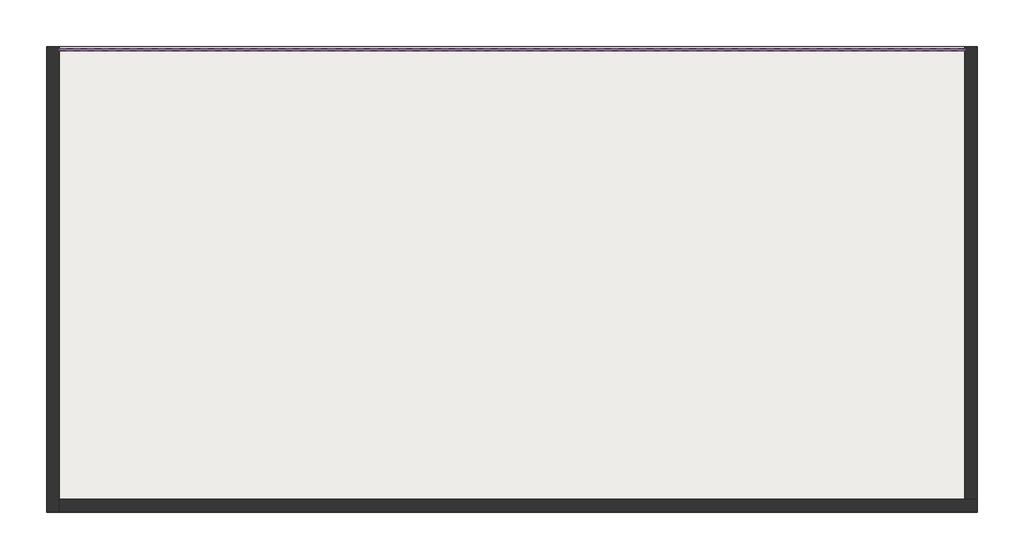
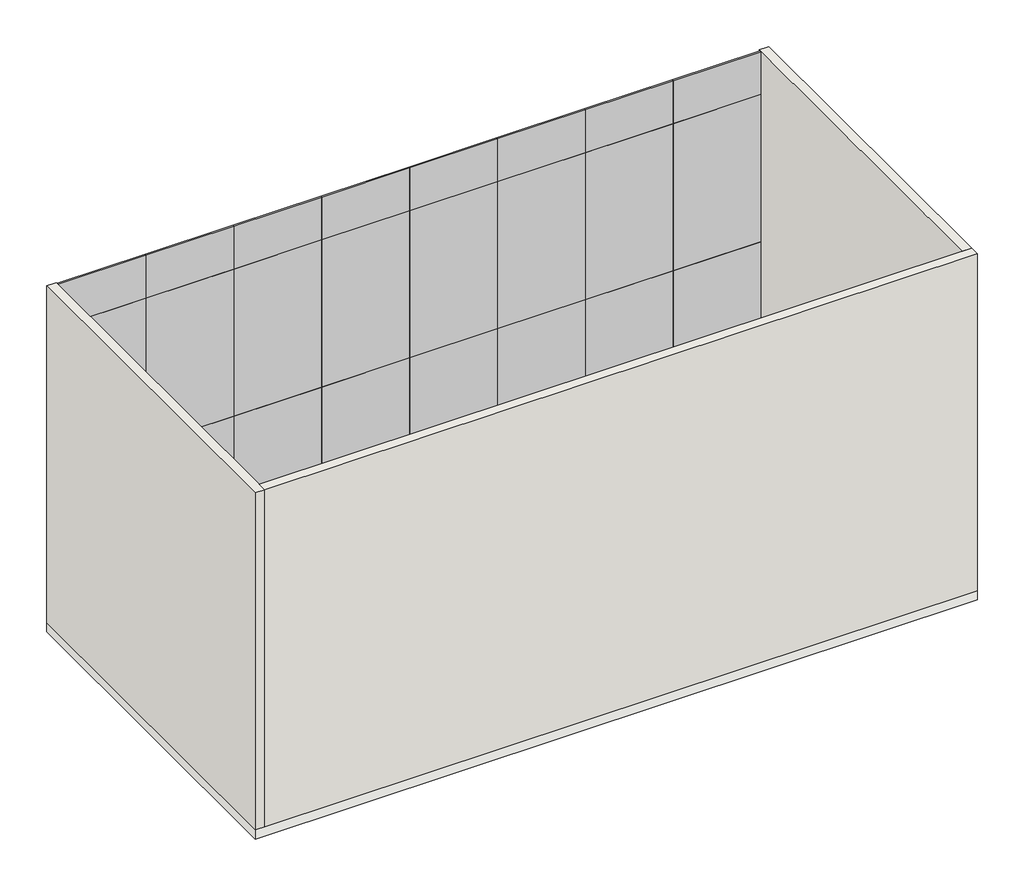
# One storey: 24 plates, 3 walls, 1 slab.
"""IFC4 building model written with IfcOpenShell, lengths in millimetres."""

import ifcopenshell
import ifcopenshell.guid

model = None  # the IFC model being written
_history = None  # IfcOwnerHistory: only IFC2X3 demands one
_inside = {}  # id of a spatial element -> (the spatial element, [elements in it])
_under = {}  # id of a project, library or spatial element -> (it, [spatial elements below it])
_declared = {}  # id of a project -> (the project, [libraries it declares])
_typed = {}  # id of a type object -> (the type object, [elements of that type])
_made_of = {}  # id of a material, layer set ... -> (it, [elements and type objects made of it])


def new_model(schema):
    """Start an empty IFC model of exactly this schema.

    Asked for "IFC4X3", IfcOpenShell would pick the latest addendum, in which some entities
    have other attributes; the version numbers below select the first issue.
    IFC2X3 requires an IfcOwnerHistory on every rooted entity: one is made here for all.
    """
    global model, _history
    if schema == "IFC4X3":
        model = ifcopenshell.file(schema_version=(4, 3, 0, 0))
    else:
        model = ifcopenshell.file(schema=schema)
    _inside.clear()
    _under.clear()
    _declared.clear()
    _typed.clear()
    _made_of.clear()
    _history = None
    if model.schema == "IFC2X3":
        org = make("IfcOrganization", Name="unknown")
        user = make(
            "IfcPersonAndOrganization",
            ThePerson=make("IfcPerson", FamilyName="unknown"),
            TheOrganization=org,
        )
        app = make(
            "IfcApplication",
            ApplicationDeveloper=org,
            Version="unknown",
            ApplicationFullName="unknown",
            ApplicationIdentifier="unknown",
        )
        _history = make(
            "IfcOwnerHistory",
            OwningUser=user,
            OwningApplication=app,
            ChangeAction="ADDED",
            CreationDate=0,
        )
    return model


def make(cls, **values):
    """One entity of the class cls with the attributes given. An attribute that is None is left unset."""
    return model.create_entity(
        cls, **{name: value for name, value in values.items() if value is not None}
    )


def rooted(cls, **values):
    """An entity with a GlobalId (a new one), such as an element, a storey or a relation."""
    return make(cls, GlobalId=ifcopenshell.guid.new(), OwnerHistory=_history, **values)


def si_unit(unit_type, name, prefix=None):
    """IfcSIUnit, for example si_unit("LENGTHUNIT", "METRE", prefix="MILLI")."""
    return make("IfcSIUnit", UnitType=unit_type, Prefix=prefix, Name=name)


def assignment(units):
    """IfcUnitAssignment: the units of a project."""
    return None if units is None else make("IfcUnitAssignment", Units=units)


def point(xyz):
    """IfcCartesianPoint."""
    return None if xyz is None else make("IfcCartesianPoint", Coordinates=xyz)


def direction(xyz):
    """IfcDirection."""
    return None if xyz is None else make("IfcDirection", DirectionRatios=xyz)


def frame(location, z_axis=None, x_axis=None):
    """IfcAxis2Placement3D, a coordinate frame: its origin and axes. An axis left out is left unset."""
    return make(
        "IfcAxis2Placement3D",
        Location=point(location),
        Axis=direction(z_axis),
        RefDirection=direction(x_axis),
    )


def origin():
    """The frame at (0, 0, 0) with its axes left unset."""
    return frame((0.0, 0.0, 0.0))


def origin_with_axes():
    """The frame at (0, 0, 0) with the z axis (0, 0, 1) and the x axis (1, 0, 0) written out."""
    return frame((0.0, 0.0, 0.0), z_axis=(0.0, 0.0, 1.0), x_axis=(1.0, 0.0, 0.0))


def place(relative_to, where):
    """IfcLocalPlacement: puts the frame where relative to a parent placement (None: the world)."""
    return make(
        "IfcLocalPlacement", PlacementRelTo=relative_to, RelativePlacement=where
    )


def context(
    kind, dimensions, precision=None, world=None, true_north=None, identifier=None
):
    """IfcGeometricRepresentationContext, for example the 3D "Model" context."""
    return make(
        "IfcGeometricRepresentationContext",
        ContextIdentifier=identifier,
        ContextType=kind,
        CoordinateSpaceDimension=dimensions,
        Precision=precision,
        WorldCoordinateSystem=world,
        TrueNorth=true_north,
    )


def project(units=None, contexts=None):
    """IfcProject with its units and contexts."""
    return rooted(
        "IfcProject",
        Name="project",
        RepresentationContexts=contexts,
        UnitsInContext=assignment(units),
    )


def spatial(cls, under=None, at=None, **own):
    """A site, building, storey or space (cls), placed at a placement, below another one or the project."""
    s = rooted(cls, ObjectPlacement=at, **own)
    if under is not None:
        _under.setdefault(under.id(), (under, []))[1].append(s)
    return s


def polyline(points):
    """IfcPolyline through the points."""
    return make("IfcPolyline", Points=[point(p) for p in points])


def outline(outer, holes=None, kind="AREA"):
    """IfcArbitraryClosedProfileDef: a profile drawn as a closed curve; with holes, ...WithVoids."""
    if holes is None:
        return make("IfcArbitraryClosedProfileDef", ProfileType=kind, OuterCurve=outer)
    return make(
        "IfcArbitraryProfileDefWithVoids",
        ProfileType=kind,
        OuterCurve=outer,
        InnerCurves=holes,
    )


def extrude(swept, where, along, depth):
    """IfcExtrudedAreaSolid: the profile swept, set in the frame where, extruded along a direction by depth."""
    return make(
        "IfcExtrudedAreaSolid",
        SweptArea=swept,
        Position=where,
        ExtrudedDirection=direction(along),
        Depth=depth,
    )


def faces_of(points, faces, orient=None, outer=None):
    """IfcFace entities. A face is a list of loops; a loop is a list of indices into points, from 0.

    orient and outer hold one flag for each loop. By default every Orientation is true, the
    first loop of a face is its IfcFaceOuterBound and the others are IfcFaceBound.
    """
    made = []
    for i, loops in enumerate(faces):
        bounds = []
        for j, loop in enumerate(loops):
            is_outer = j == 0 if outer is None else outer[i][j]
            bounds.append(
                make(
                    "IfcFaceOuterBound" if is_outer else "IfcFaceBound",
                    Bound=make("IfcPolyLoop", Polygon=[points[k] for k in loop]),
                    Orientation=True if orient is None else orient[i][j],
                )
            )
        made.append(make("IfcFace", Bounds=bounds))
    return made


def faceted_brep(points, faces, orient=None, outer=None, voids=None):
    """IfcFacetedBrep: a solid bounded by flat faces; with voids (closed shells), ...WithVoids."""
    shared = [point(p) for p in points]
    hull = make("IfcClosedShell", CfsFaces=faces_of(shared, faces, orient, outer))
    if voids is None:
        return make("IfcFacetedBrep", Outer=hull)
    return make(
        "IfcFacetedBrepWithVoids",
        Outer=hull,
        Voids=[
            make(cls, CfsFaces=faces_of(shared, fs, o, b)) for cls, fs, o, b in voids
        ],
    )


def shape(context_of_items, identifier, shape_type, items):
    """IfcShapeRepresentation: the items that make up one representation, for example the "Body"."""
    return make(
        "IfcShapeRepresentation",
        ContextOfItems=context_of_items,
        RepresentationIdentifier=identifier,
        RepresentationType=shape_type,
        Items=items,
    )


def source(mapping_origin, context_of_items, identifier, shape_type, items):
    """IfcRepresentationMap: a shape defined once, which mapped items show again and again."""
    return make(
        "IfcRepresentationMap",
        MappingOrigin=mapping_origin,
        MappedRepresentation=shape(context_of_items, identifier, shape_type, items),
    )


def transform(
    local_origin,
    x_axis=None,
    y_axis=None,
    z_axis=None,
    scale=None,
    scale2=None,
    scale3=None,
    uniform=True,
):
    """IfcCartesianTransformationOperator3D, or its non-uniform kind. x_axis, y_axis, z_axis: its Axis1, 2, 3."""
    if uniform:
        return make(
            "IfcCartesianTransformationOperator3D",
            Axis1=direction(x_axis),
            Axis2=direction(y_axis),
            LocalOrigin=point(local_origin),
            Scale=scale,
            Axis3=direction(z_axis),
        )
    return make(
        "IfcCartesianTransformationOperator3DnonUniform",
        Axis1=direction(x_axis),
        Axis2=direction(y_axis),
        LocalOrigin=point(local_origin),
        Scale=scale,
        Axis3=direction(z_axis),
        Scale2=scale2,
        Scale3=scale3,
    )


def mapped(mapping_source, mapping_target):
    """IfcMappedItem: shows the shape of a source again, moved by a transform."""
    return make(
        "IfcMappedItem", MappingSource=mapping_source, MappingTarget=mapping_target
    )


def made_of(thing, what):
    """Note that an element or type object is made of a material, layer set ...; save() writes the relation."""
    if what is not None:
        _made_of.setdefault(what.id(), (what, []))[1].append(thing)
    return thing


def element(
    cls,
    number,
    at=None,
    inside=None,
    cuts=None,
    type_object=None,
    material=None,
    context=None,
    identifier="Body",
    shape_type=None,
    held_by="IfcProductDefinitionShape",
    body=None,
    shapes=None,
    **own,
):
    """One element of the class cls, such as IfcWall. Its Tag is "e" and its number.

    at: its placement. inside: the storey or other place that contains it. cuts: it is an
    opening in that element (IfcRelVoidsElement). A single representation is given by context,
    identifier, shape_type and body (its items); several are given by shapes. held_by: the class
    of the entity that holds the representations. save() writes the other relations.
    """
    e = rooted(cls, Tag="e%d" % number, ObjectPlacement=at, **own)
    if body is not None:
        shapes = [shape(context, identifier, shape_type, body)]
    if shapes is not None:
        e.Representation = make(held_by, Representations=shapes)
    if inside is not None:
        _inside.setdefault(inside.id(), (inside, []))[1].append(e)
    if cuts is not None:
        rooted(
            "IfcRelVoidsElement", RelatingBuildingElement=cuts, RelatedOpeningElement=e
        )
    if type_object is not None:
        _typed.setdefault(type_object.id(), (type_object, []))[1].append(e)
    return made_of(e, material)


def aggregate(whole, parts):
    """IfcRelAggregates: a whole, such as a stair, and the parts it consists of."""
    return rooted("IfcRelAggregates", RelatingObject=whole, RelatedObjects=parts)


def save(model, path):
    """Write the relations noted so far, then the file.

    IfcRelAggregates (storeys below a building ...), IfcRelContainedInSpatialStructure (elements
    in a storey), IfcRelDefinesByType, IfcRelAssociatesMaterial and IfcRelDeclares: one each for
    every whole, place, type object, material and project.
    """
    for whole, parts in _under.values():
        aggregate(whole, parts)
    for where, things in _inside.values():
        rooted(
            "IfcRelContainedInSpatialStructure",
            RelatedElements=things,
            RelatingStructure=where,
        )
    for kind, things in _typed.values():
        rooted("IfcRelDefinesByType", RelatedObjects=things, RelatingType=kind)
    for what, things in _made_of.values():
        rooted("IfcRelAssociatesMaterial", RelatedObjects=things, RelatingMaterial=what)
    for by, libraries in _declared.values():
        rooted("IfcRelDeclares", RelatingContext=by, RelatedDefinitions=libraries)
    model.write(path)


def plate_c1c025ea(model_context):
    return source(origin(), model_context, "Body", "SweptSolid", [
        extrude(outline(polyline([(678.1250001, 24.5), (-678.1250001, 24.5), (-678.1250001, 49.5), (678.1250001, 49.5), (678.1250001, 24.5)])), origin_with_axes(), (0.0, 0.0, 1.0), 2400.0),
    ])


def plate_0eebf7e9(model_context):
    return source(origin(), model_context, "Body", "SweptSolid", [
        extrude(outline(polyline([(678.1250001, 24.5), (-678.1250001, 24.5), (-678.1250001, 49.5), (678.1250001, 49.5), (678.1250001, 24.5)])), origin_with_axes(), (0.0, 0.0, 1.0), 700.0),
    ])


model = new_model("IFC4")

# Units and contexts
model_context = context("Model", 3, world=origin())
ifc_project = project(units=[si_unit("LENGTHUNIT", "METRE", prefix="MILLI")], contexts=[model_context])

# Site, building, storey
site = spatial("IfcSite", under=ifc_project)
building = spatial("IfcBuilding", under=site)
storey = spatial("IfcBuildingStorey", under=building, Name="レベル 1", Elevation=500.0)

# Plates
placement = place(None, origin())
plate_shape = plate_c1c025ea(model_context)
element("IfcPlate", 1, ObjectType="システム パネル : ガラス", at=placement, inside=storey, context=model_context, shape_type="MappedRepresentation", body=[
    mapped(plate_shape, transform((2064.186127, 4477.4867718, 500.0), x_axis=(-1.0, 0.0, 0.0), y_axis=(0.0, -1.0, 0.0), z_axis=(0.0, 0.0, 1.0))),
])
element("IfcPlate", 2, ObjectType="システム パネル : ガラス", at=placement, inside=storey, context=model_context, shape_type="MappedRepresentation", body=[
    mapped(plate_shape, transform((707.9361269, 4477.4867718, 500.0), x_axis=(-1.0, 0.0, 0.0), y_axis=(0.0, -1.0, 0.0), z_axis=(0.0, 0.0, 1.0))),
])
element("IfcPlate", 3, ObjectType="システム パネル : ガラス", at=placement, inside=storey, context=model_context, shape_type="MappedRepresentation", body=[
    mapped(plate_shape, transform((-648.313873, 4477.4867718, 500.0), x_axis=(-1.0, 0.0, 0.0), y_axis=(0.0, -1.0, 0.0), z_axis=(0.0, 0.0, 1.0))),
])
element("IfcPlate", 4, ObjectType="システム パネル : ガラス", at=placement, inside=storey, context=model_context, shape_type="MappedRepresentation", body=[
    mapped(plate_shape, transform((-2004.5638729, 4477.4867718, 500.0), x_axis=(-1.0, 0.0, 0.0), y_axis=(0.0, -1.0, 0.0), z_axis=(0.0, 0.0, 1.0))),
])
element("IfcPlate", 5, ObjectType="システム パネル : ガラス", at=placement, inside=storey, context=model_context, shape_type="MappedRepresentation", body=[
    mapped(plate_shape, transform((-3360.8138728, 4477.4867718, 500.0), x_axis=(-1.0, 0.0, 0.0), y_axis=(0.0, -1.0, 0.0), z_axis=(0.0, 0.0, 1.0))),
])
element("IfcPlate", 6, ObjectType="システム パネル : ガラス", at=placement, inside=storey, context=model_context, shape_type="MappedRepresentation", body=[
    mapped(plate_shape, transform((-4717.0638727, 4477.4867718, 500.0), x_axis=(-1.0, 0.0, 0.0), y_axis=(0.0, -1.0, 0.0), z_axis=(0.0, 0.0, 1.0))),
])
element("IfcPlate", 7, ObjectType="システム パネル : ガラス", at=placement, inside=storey, context=model_context, shape_type="MappedRepresentation", body=[
    mapped(plate_shape, transform((-6073.3138727, 4477.4867718, 500.0), x_axis=(-1.0, 0.0, 0.0), y_axis=(0.0, -1.0, 0.0), z_axis=(0.0, 0.0, 1.0))),
])
element("IfcPlate", 8, ObjectType="システム パネル : ガラス", at=placement, inside=storey, context=model_context, shape_type="MappedRepresentation", body=[
    mapped(plate_shape, transform((-7429.5638727, 4477.4867718, 500.0), x_axis=(-1.0, 0.0, 0.0), y_axis=(0.0, -1.0, 0.0), z_axis=(0.0, 0.0, 1.0))),
])
element("IfcPlate", 9, ObjectType="システム パネル : ガラス", at=placement, inside=storey, context=model_context, shape_type="MappedRepresentation", body=[
    mapped(plate_shape, transform((2064.186127, 4477.4867718, 2900.0), x_axis=(-1.0, 0.0, 0.0), y_axis=(0.0, -1.0, 0.0), z_axis=(0.0, 0.0, 1.0))),
])
element("IfcPlate", 10, ObjectType="システム パネル : ガラス", at=placement, inside=storey, context=model_context, shape_type="MappedRepresentation", body=[
    mapped(plate_shape, transform((707.9361269, 4477.4867718, 2900.0), x_axis=(-1.0, 0.0, 0.0), y_axis=(0.0, -1.0, 0.0), z_axis=(0.0, 0.0, 1.0))),
])
element("IfcPlate", 11, ObjectType="システム パネル : ガラス", at=placement, inside=storey, context=model_context, shape_type="MappedRepresentation", body=[
    mapped(plate_shape, transform((-648.313873, 4477.4867718, 2900.0), x_axis=(-1.0, 0.0, 0.0), y_axis=(0.0, -1.0, 0.0), z_axis=(0.0, 0.0, 1.0))),
])
element("IfcPlate", 12, ObjectType="システム パネル : ガラス", at=placement, inside=storey, context=model_context, shape_type="MappedRepresentation", body=[
    mapped(plate_shape, transform((-2004.5638729, 4477.4867718, 2900.0), x_axis=(-1.0, 0.0, 0.0), y_axis=(0.0, -1.0, 0.0), z_axis=(0.0, 0.0, 1.0))),
])
element("IfcPlate", 13, ObjectType="システム パネル : ガラス", at=placement, inside=storey, context=model_context, shape_type="MappedRepresentation", body=[
    mapped(plate_shape, transform((-3360.8138728, 4477.4867718, 2900.0), x_axis=(-1.0, 0.0, 0.0), y_axis=(0.0, -1.0, 0.0), z_axis=(0.0, 0.0, 1.0))),
])
element("IfcPlate", 14, ObjectType="システム パネル : ガラス", at=placement, inside=storey, context=model_context, shape_type="MappedRepresentation", body=[
    mapped(plate_shape, transform((-4717.0638727, 4477.4867718, 2900.0), x_axis=(-1.0, 0.0, 0.0), y_axis=(0.0, -1.0, 0.0), z_axis=(0.0, 0.0, 1.0))),
])
element("IfcPlate", 15, ObjectType="システム パネル : ガラス", at=placement, inside=storey, context=model_context, shape_type="MappedRepresentation", body=[
    mapped(plate_shape, transform((-6073.3138727, 4477.4867718, 2900.0), x_axis=(-1.0, 0.0, 0.0), y_axis=(0.0, -1.0, 0.0), z_axis=(0.0, 0.0, 1.0))),
])
element("IfcPlate", 16, ObjectType="システム パネル : ガラス", at=placement, inside=storey, context=model_context, shape_type="MappedRepresentation", body=[
    mapped(plate_shape, transform((-7429.5638727, 4477.4867718, 2900.0), x_axis=(-1.0, 0.0, 0.0), y_axis=(0.0, -1.0, 0.0), z_axis=(0.0, 0.0, 1.0))),
])
plate_2_shape = plate_0eebf7e9(model_context)
element("IfcPlate", 17, ObjectType="システム パネル : ガラス", at=placement, inside=storey, context=model_context, shape_type="MappedRepresentation", body=[
    mapped(plate_2_shape, transform((2064.186127, 4477.4867718, 5300.0), x_axis=(-1.0, 0.0, 0.0), y_axis=(0.0, -1.0, 0.0), z_axis=(0.0, 0.0, 1.0))),
])
element("IfcPlate", 18, ObjectType="システム パネル : ガラス", at=placement, inside=storey, context=model_context, shape_type="MappedRepresentation", body=[
    mapped(plate_2_shape, transform((707.9361269, 4477.4867718, 5300.0), x_axis=(-1.0, 0.0, 0.0), y_axis=(0.0, -1.0, 0.0), z_axis=(0.0, 0.0, 1.0))),
])
element("IfcPlate", 19, ObjectType="システム パネル : ガラス", at=placement, inside=storey, context=model_context, shape_type="MappedRepresentation", body=[
    mapped(plate_2_shape, transform((-648.313873, 4477.4867718, 5300.0), x_axis=(-1.0, 0.0, 0.0), y_axis=(0.0, -1.0, 0.0), z_axis=(0.0, 0.0, 1.0))),
])
element("IfcPlate", 20, ObjectType="システム パネル : ガラス", at=placement, inside=storey, context=model_context, shape_type="MappedRepresentation", body=[
    mapped(plate_2_shape, transform((-2004.5638729, 4477.4867718, 5300.0), x_axis=(-1.0, 0.0, 0.0), y_axis=(0.0, -1.0, 0.0), z_axis=(0.0, 0.0, 1.0))),
])
element("IfcPlate", 21, ObjectType="システム パネル : ガラス", at=placement, inside=storey, context=model_context, shape_type="MappedRepresentation", body=[
    mapped(plate_2_shape, transform((-3360.8138728, 4477.4867718, 5300.0), x_axis=(-1.0, 0.0, 0.0), y_axis=(0.0, -1.0, 0.0), z_axis=(0.0, 0.0, 1.0))),
])
element("IfcPlate", 22, ObjectType="システム パネル : ガラス", at=placement, inside=storey, context=model_context, shape_type="MappedRepresentation", body=[
    mapped(plate_2_shape, transform((-4717.0638727, 4477.4867718, 5300.0), x_axis=(-1.0, 0.0, 0.0), y_axis=(0.0, -1.0, 0.0), z_axis=(0.0, 0.0, 1.0))),
])
element("IfcPlate", 23, ObjectType="システム パネル : ガラス", at=placement, inside=storey, context=model_context, shape_type="MappedRepresentation", body=[
    mapped(plate_2_shape, transform((-6073.3138727, 4477.4867718, 5300.0), x_axis=(-1.0, 0.0, 0.0), y_axis=(0.0, -1.0, 0.0), z_axis=(0.0, 0.0, 1.0))),
])
element("IfcPlate", 24, ObjectType="システム パネル : ガラス", at=placement, inside=storey, context=model_context, shape_type="MappedRepresentation", body=[
    mapped(plate_2_shape, transform((-7429.5638727, 4477.4867718, 5300.0), x_axis=(-1.0, 0.0, 0.0), y_axis=(0.0, -1.0, 0.0), z_axis=(0.0, 0.0, 1.0))),
])

# Slab
element("IfcSlab", 25, ObjectType="一般 150 mm", at=placement, inside=storey, context=model_context, shape_type="SweptSolid", body=[
    extrude(outline(polyline([(2892.3111271, 4477.4867718), (2892.3111271, -1097.5132282), (-8257.6888729, -1097.5132282), (-8257.6888729, 4477.4867718), (2892.3111271, 4477.4867718)])), frame((0.0, 0.0, 350.0), z_axis=(0.0, 0.0, 1.0), x_axis=(1.0, 0.0, 0.0)), (0.0, 0.0, 1.0), 150.0),
])

# Walls
element("IfcWall", 26, ObjectType="GEL-Wall-150mm", at=placement, inside=storey, context=model_context, shape_type="Brep", body=[
    faceted_brep([(-8257.6888729, 4477.4867718, 500.0), (-8257.6888729, -1097.5132282, 500.0), (-8257.6888729, -1097.5132282, 6000.0), (-8257.6888729, 4477.4867718, 6000.0), (-8107.6888729, 4477.4867718, 500.0), (-8107.6888729, 4477.4867718, 6000.0), (-8107.6888729, -947.5132282, 6000.0), (-8107.6888729, -1097.5132282, 6000.0), (-8107.6888729, -1097.5132282, 500.0), (-8107.6888729, -947.5132282, 500.0)], [[[0, 1, 2, 3]], [[4, 5, 6, 7, 8, 9]], [[1, 0, 4, 9, 8]], [[3, 2, 7, 6, 5]], [[0, 3, 5, 4]], [[2, 1, 8, 7]]]),
])
element("IfcWall", 27, ObjectType="GEL-Wall-150mm", at=placement, inside=storey, context=model_context, shape_type="Brep", body=[
    faceted_brep([(-8107.6888729, -1097.5132282, 500.0), (2892.3111271, -1097.5132282, 500.0), (2892.3111271, -1097.5132282, 6000.0), (-8107.6888729, -1097.5132282, 6000.0), (-8107.6888729, -947.5132282, 500.0), (-8107.6888729, -947.5132282, 6000.0), (2742.3111271, -947.5132282, 6000.0), (2892.3111271, -947.5132282, 6000.0), (2892.3111271, -947.5132282, 500.0), (2742.3111271, -947.5132282, 500.0)], [[[0, 1, 2, 3]], [[4, 5, 6, 7, 8, 9]], [[1, 0, 4, 9, 8]], [[3, 2, 7, 6, 5]], [[0, 3, 5, 4]], [[2, 1, 8, 7]]]),
])
element("IfcWall", 28, ObjectType="GEL-Wall-150mm", at=placement, inside=storey, context=model_context, shape_type="SweptSolid", body=[
    extrude(outline(polyline([(2892.3111271, 4477.4867718), (2892.3111271, -947.5132282), (2742.3111271, -947.5132282), (2742.3111271, 4477.4867718), (2892.3111271, 4477.4867718)])), frame((0.0, 0.0, 500.0), z_axis=(0.0, 0.0, 1.0), x_axis=(1.0, 0.0, 0.0)), (0.0, 0.0, 1.0), 5500.0),
])

save(model, "model.ifc")

# Revit data of these elements
# Project information
#   プロジェクト発行日 = "発行日"
#   プロジェクト ステータス = "プロジェクト ステータス"
#   クライアント名 = "オーナ"
#   計画地住所 = "ここにアドレスを入力"
#   プロジェクト名 = "プロジェクト名"
#   プロジェクト番号 = "0001"
# Type "システム パネル : ガラス"
#   Construction Type Id = "GSP4R"
#   Analytic Construction = "1/8 インチ ピルキントン一重ガラス"
#   Visual Light Transmittance = 0.9
#   Solar Heat Gain Coefficient = 0.86
#   Heat Transfer Coefficient (U) = 6.7069 W/(m²·K)
# Type "一般 150 mm"
#   Function = 0
#   Layers, outside or top first: 150 mm no material (function 1)
# Type "GEL-Wall-150mm"
#   Layers, outside or top first: 150 mm "Off-White Plaster" (function 1)
# Elements 1, 2, 3, 4, 5, 6, 7, 8, 9, 10, 11, 12, 13, 14, 15, 16, 17, 18, 19, 20, 21, 22, 23, 24 (IfcPlate, "システム パネル : ガラス")
#   Phase Created = 新しい建設
#   Materials on its faces: "ガラス - 透明"
# Element 25 (IfcSlab, "一般 150 mm")
#   Height Offset From Level = 0 mm
#   Phase Created = 新しい建設
# Elements 26, 27, 28 (IfcWall, "GEL-Wall-150mm")
#   Top Offset = 0 mm
#   Base Offset = 0 mm
#   wall height = 5500 mm
#   Phase Created = 新しい建設
#   Base Constraint = レベル 1
#   Top Constraint = レベル 2
#   Materials on its faces: "Off-White Plaster"
# Materials
#   "Off-White Plaster": class "一般", colour RGB 236 238 235, transparency 0, Cost = 0
#   "ガラス - 透明": class "ガラス", colour RGB 0 128 192, transparency 0.9, Cost = 0
# Room at (-2327.994, 1835.329) mm, phase "新しい建設", upper level "レベル 1", upper offset 3500 mm, lower offset 0 mm
#   Number = "1"
#   Name = "部屋"
